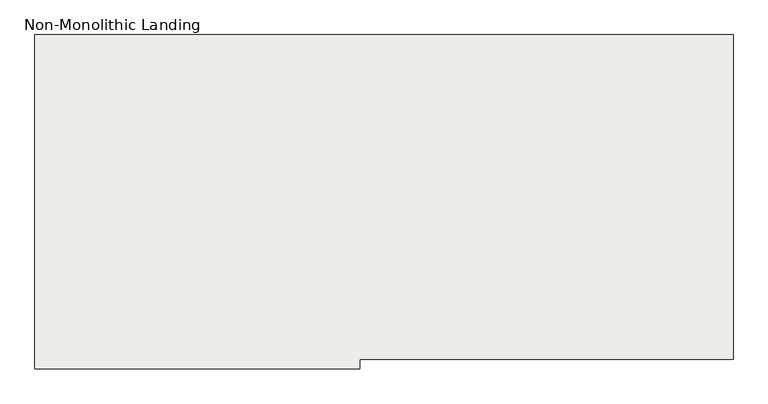
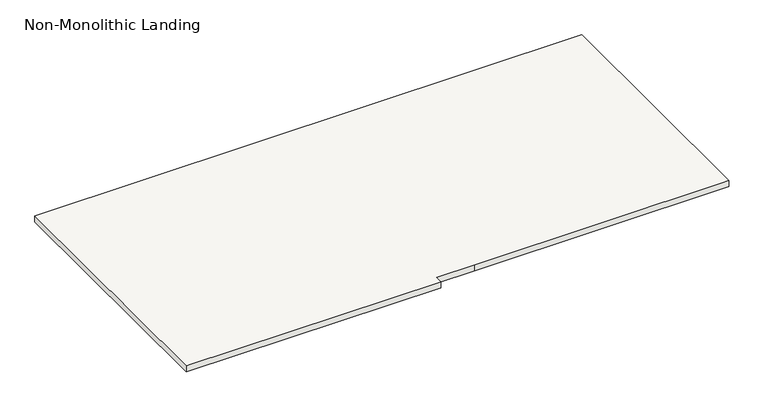
"""IFC4 building model written with IfcOpenShell, lengths in millimetres: slab geometry, Non-Monolithic Landing."""

from ifc_helpers import new_model, si_unit, frame, origin, place, context, project, spatial, polyline, outline, extrude, source, transform, mapped, element, save


def non_monolithic_landing_caa1b051(model_context):
    return source(origin(), model_context, "Body", "SweptSolid", [
        extrude(outline(polyline([(12700.0002443, 23469.9999999), (12700.0002443, 25529.9999999), (17000.0002442, 25529.9999999), (17000.0002442, 23529.9999999), (15000.0002442, 23529.9999999), (14700.0002443, 23529.9999999), (14700.0002443, 23469.9999999), (12700.0002443, 23469.9999999)])), frame((0.0, 0.0, 27783.3333333), z_axis=(0.0, 0.0, 1.0), x_axis=(1.0, 0.0, 0.0)), (0.0, 0.0, 1.0), 50.0),
    ])


if __name__ == "__main__":
    model = new_model("IFC4")
    model_context = context("Model", 3, world=origin())
    ifc_project = project(units=[si_unit("LENGTHUNIT", "METRE", prefix="MILLI")], contexts=[model_context])
    site = spatial("IfcSite", under=ifc_project)
    building = spatial("IfcBuilding", under=site)
    placement = place(None, origin())
    non_monolithic_landing_shape = non_monolithic_landing_caa1b051(model_context)
    element("IfcSlab", 1, ObjectType="Non-Monolithic Landing", at=placement, inside=building, context=model_context, shape_type="MappedRepresentation", body=[
        mapped(non_monolithic_landing_shape, transform((0.0, 0.0, 0.0), x_axis=(1.0, 0.0, 0.0), y_axis=(0.0, 1.0, 0.0), z_axis=(0.0, 0.0, 1.0))),
    ])
    save(model, "model.ifc")
